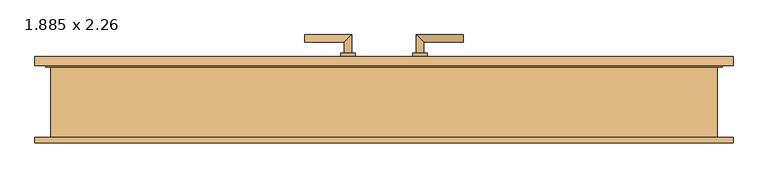
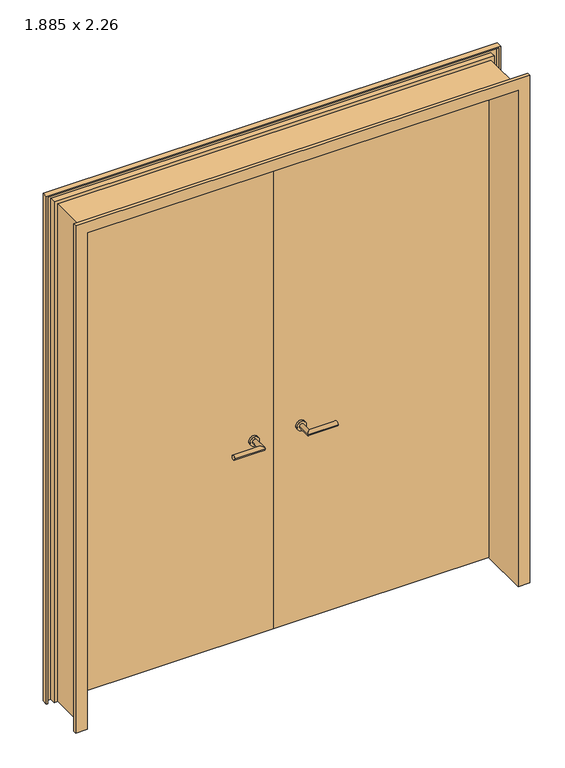
"""IFC4 building model written with IfcOpenShell, lengths in millimetres: door geometry, Drehflügel 2-flg - Stahlzarge : 1.885 x 2.26."""

from ifc_helpers import new_model, si_unit, point, frame, frame_2d, origin, place, context, project, spatial, polyline, circle_curve, ellipse_curve, trimmed, segment, composite_curve, outline, extrude, faceted_brep, source, transform, mapped, element, save
from ifc_brep_helpers import plane_surface, cylinder_surface, advanced_brep


def door_1_885_x_2_26_dae8c6c6(model_context):
    return source(origin(), model_context, "Body", "SolidModel", [
        advanced_brep(
        [(-90.0, 89.4346141, 1000.0), (-110.0, 89.4346141, 1000.0), (-110.0, 39.4346141, 1000.0), (-90.0, 19.4346141, 1000.0), (-220.0, 19.4346141, 1000.0), (-220.0, 39.4346141, 1000.0)],
        [
            (0, 1, circle_curve(frame((-100.0, 89.4346141, 1000.0), z_axis=(0.0, 1.0, 0.0), x_axis=(-1.0, 0.0, 0.0)), 10.0)),
            (1, 0, circle_curve(frame((-100.0, 89.4346141, 1000.0), z_axis=(0.0, 1.0, 0.0), x_axis=(-1.0, 0.0, 0.0)), 10.0)),
            (1, 2),
            (2, 3, ellipse_curve(frame((-100.0, 29.4346141, 1000.0), z_axis=(0.7071067811865385, 0.7071067811865565, 0.0), x_axis=(-0.7071067811865563, 0.7071067811865386, 0.0)), 14.1421356, 10.0)),
            (3, 0),
            (3, 2, ellipse_curve(frame((-100.0, 29.4346141, 1000.0), z_axis=(0.7071067811865385, 0.7071067811865565, 0.0), x_axis=(-0.7071067811865563, 0.7071067811865386, 0.0)), 14.1421356, 10.0)),
            (4, 5, circle_curve(frame((-220.0, 29.4346141, 1000.0), z_axis=(-1.0, 0.0, 0.0), x_axis=(0.0, 1.0, 0.0)), 10.0)),
            (5, 4, circle_curve(frame((-220.0, 29.4346141, 1000.0), z_axis=(-1.0, 0.0, 0.0), x_axis=(0.0, 1.0, 0.0)), 10.0)),
            (2, 5),
            (4, 3),
        ],
        [
            plane_surface(frame((-100.0, 89.4346141, -287.7526403), z_axis=(0.0, 1.0, 0.0), x_axis=(0.0, 0.0, 1.0))),
            cylinder_surface(frame((-100.0, 89.4346141, 1000.0), z_axis=(0.0, 1.0, 0.0), x_axis=(-1.0, 0.0, 0.0)), 10.0),
            plane_surface(frame((-220.0, 29.4346141, -287.7526403), z_axis=(-1.0, 0.0, 0.0), x_axis=(0.0, 0.0, 1.0))),
            cylinder_surface(frame((-100.0, 29.4346141, 1000.0), z_axis=(1.0, 0.0, 0.0), x_axis=(0.0, 1.0, 0.0)), 10.0),
        ],
        [
            (0, [[1, 2]]),
            (1, [[3, 4, 5, -2]]),
            (1, [[-5, 6, -3, -1]]),
            (2, [[7, 8]]),
            (3, [[9, -7, 10, -4]]),
            (3, [[-10, -8, -9, -6]]),
        ],
    ),
        advanced_brep(
        [(-110.0, 149.4346141, 1000.0), (-90.0, 149.4346141, 1000.0), (-90.0, 199.4346141, 1000.0), (-110.0, 179.4346141, 1000.0), (-220.0, 179.4346141, 1000.0), (-220.0, 199.4346141, 1000.0)],
        [
            (0, 1, circle_curve(frame((-100.0, 149.4346141, 1000.0), z_axis=(0.0, -1.0, 0.0), x_axis=(1.0, 0.0, 0.0)), 10.0)),
            (1, 0, circle_curve(frame((-100.0, 149.4346141, 1000.0), z_axis=(0.0, -1.0, 0.0), x_axis=(1.0, 0.0, 0.0)), 10.0)),
            (1, 2),
            (2, 3, ellipse_curve(frame((-100.0, 189.4346141, 1000.0), z_axis=(0.7071067811865475, -0.7071067811865475, 0.0), x_axis=(-0.7071067811865474, -0.7071067811865476, 0.0)), 14.1421356, 10.0)),
            (3, 0),
            (3, 2, ellipse_curve(frame((-100.0, 189.4346141, 1000.0), z_axis=(0.7071067811865475, -0.7071067811865475, 0.0), x_axis=(-0.7071067811865474, -0.7071067811865476, 0.0)), 14.1421356, 10.0)),
            (4, 5, circle_curve(frame((-220.0, 189.4346141, 1000.0), z_axis=(-1.0, 0.0, 0.0), x_axis=(0.0, 1.0, 0.0)), 10.0)),
            (5, 4, circle_curve(frame((-220.0, 189.4346141, 1000.0), z_axis=(-1.0, 0.0, 0.0), x_axis=(0.0, 1.0, 0.0)), 10.0)),
            (2, 5),
            (4, 3),
        ],
        [
            plane_surface(frame((-100.0, 149.4346141, -287.7526403), z_axis=(0.0, -1.0, 0.0), x_axis=(0.0, 0.0, 1.0))),
            cylinder_surface(frame((-100.0, 149.4346141, 1000.0), z_axis=(0.0, -1.0, 0.0), x_axis=(1.0, 0.0, 0.0)), 10.0),
            plane_surface(frame((-220.0, 189.4346141, -287.7526403), z_axis=(-1.0, 0.0, 0.0), x_axis=(0.0, 0.0, 1.0))),
            cylinder_surface(frame((-100.0, 189.4346141, 1000.0), z_axis=(1.0, 0.0, 0.0), x_axis=(0.0, 1.0, 0.0)), 10.0),
        ],
        [
            (0, [[1, 2]]),
            (1, [[3, 4, 5, -2]]),
            (1, [[-5, 6, -3, -1]]),
            (2, [[7, 8]]),
            (3, [[9, -7, 10, -4]]),
            (3, [[-10, -8, -9, -6]]),
        ],
    ),
        extrude(outline(composite_curve([segment(trimmed(circle_curve(frame_2d((1000.0, -100.0)), 20.0), [point((1000.0, -80.0))], [point((1000.0, -120.0))], False, "CARTESIAN"), True, "CONTINUOUS"), segment(trimmed(circle_curve(frame_2d((1000.0, -100.0)), 20.0), [point((1000.0, -120.0))], [point((1000.0, -80.0))], False, "CARTESIAN"), True, "CONTINUOUS")], self_intersect=False)), frame((0.0, 79.4346141, 0.0), z_axis=(0.0, 1.0, 0.0), x_axis=(0.0, 0.0, 1.0)), (0.0, 0.0, 1.0), 10.0),
        extrude(outline(composite_curve([segment(trimmed(circle_curve(frame_2d((1000.0, -100.0)), 20.0), [point((1000.0, -80.0))], [point((1000.0, -120.0))], False, "CARTESIAN"), True, "CONTINUOUS"), segment(trimmed(circle_curve(frame_2d((1000.0, -100.0)), 20.0), [point((1000.0, -120.0))], [point((1000.0, -80.0))], False, "CARTESIAN"), True, "CONTINUOUS")], self_intersect=False)), frame((0.0, 139.4346141, 0.0), z_axis=(0.0, 1.0, 0.0), x_axis=(0.0, 0.0, 1.0)), (0.0, 0.0, 1.0), 10.0),
        advanced_brep(
        [(90.0, 89.4346141, 1000.0), (110.0, 89.4346141, 1000.0), (90.0, 19.4346141, 1000.0), (110.0, 39.4346141, 1000.0), (220.0, 19.4346141, 1000.0), (220.0, 39.4346141, 1000.0)],
        [
            (0, 1, circle_curve(frame((100.0, 89.4346141, 1000.0), z_axis=(0.0, 1.0, 0.0), x_axis=(1.0, 0.0, 0.0)), 10.0)),
            (1, 0, circle_curve(frame((100.0, 89.4346141, 1000.0), z_axis=(0.0, 1.0, 0.0), x_axis=(1.0, 0.0, 0.0)), 10.0)),
            (0, 2),
            (2, 3, ellipse_curve(frame((100.0, 29.4346141, 1000.0), z_axis=(-0.7071067811865385, 0.7071067811865565, 0.0), x_axis=(0.7071067811865563, 0.7071067811865386, 0.0)), 14.1421356, 10.0)),
            (3, 1),
            (3, 2, ellipse_curve(frame((100.0, 29.4346141, 1000.0), z_axis=(-0.7071067811865385, 0.7071067811865565, 0.0), x_axis=(0.7071067811865563, 0.7071067811865386, 0.0)), 14.1421356, 10.0)),
            (4, 5, circle_curve(frame((220.0, 29.4346141, 1000.0), z_axis=(1.0, 0.0, 0.0), x_axis=(0.0, 1.0, 0.0)), 10.0)),
            (5, 4, circle_curve(frame((220.0, 29.4346141, 1000.0), z_axis=(1.0, 0.0, 0.0), x_axis=(0.0, 1.0, 0.0)), 10.0)),
            (2, 4),
            (5, 3),
        ],
        [
            plane_surface(frame((100.0, 89.4346141, -287.7526403), z_axis=(0.0, 1.0, 0.0), x_axis=(0.0, 0.0, 1.0))),
            cylinder_surface(frame((100.0, 89.4346141, 1000.0), z_axis=(0.0, 1.0, 0.0), x_axis=(1.0, 0.0, 0.0)), 10.0),
            plane_surface(frame((220.0, 29.4346141, -287.7526403), z_axis=(1.0, 0.0, 0.0), x_axis=(0.0, 0.0, 1.0))),
            cylinder_surface(frame((100.0, 29.4346141, 1000.0), z_axis=(-1.0, 0.0, 0.0), x_axis=(0.0, 1.0, 0.0)), 10.0),
        ],
        [
            (0, [[1, 2]]),
            (1, [[-1, 3, 4, 5]]),
            (1, [[-2, -5, 6, -3]]),
            (2, [[7, 8]]),
            (3, [[-4, 9, -8, 10]]),
            (3, [[-6, -10, -7, -9]]),
        ],
    ),
        advanced_brep(
        [(110.0, 149.4346141, 1000.0), (90.0, 149.4346141, 1000.0), (110.0, 179.4346141, 1000.0), (90.0, 199.4346141, 1000.0), (220.0, 179.4346141, 1000.0), (220.0, 199.4346141, 1000.0)],
        [
            (0, 1, circle_curve(frame((100.0, 149.4346141, 1000.0), z_axis=(0.0, -1.0, 0.0), x_axis=(-1.0, 0.0, 0.0)), 10.0)),
            (1, 0, circle_curve(frame((100.0, 149.4346141, 1000.0), z_axis=(0.0, -1.0, 0.0), x_axis=(-1.0, 0.0, 0.0)), 10.0)),
            (0, 2),
            (2, 3, ellipse_curve(frame((100.0, 189.4346141, 1000.0), z_axis=(-0.7071067811865475, -0.7071067811865475, 0.0), x_axis=(0.7071067811865474, -0.7071067811865476, 0.0)), 14.1421356, 10.0)),
            (3, 1),
            (3, 2, ellipse_curve(frame((100.0, 189.4346141, 1000.0), z_axis=(-0.7071067811865475, -0.7071067811865475, 0.0), x_axis=(0.7071067811865474, -0.7071067811865476, 0.0)), 14.1421356, 10.0)),
            (4, 5, circle_curve(frame((220.0, 189.4346141, 1000.0), z_axis=(1.0, 0.0, 0.0), x_axis=(0.0, 1.0, 0.0)), 10.0)),
            (5, 4, circle_curve(frame((220.0, 189.4346141, 1000.0), z_axis=(1.0, 0.0, 0.0), x_axis=(0.0, 1.0, 0.0)), 10.0)),
            (2, 4),
            (5, 3),
        ],
        [
            plane_surface(frame((100.0, 149.4346141, -287.7526403), z_axis=(0.0, -1.0, 0.0), x_axis=(0.0, 0.0, 1.0))),
            cylinder_surface(frame((100.0, 149.4346141, 1000.0), z_axis=(0.0, -1.0, 0.0), x_axis=(-1.0, 0.0, 0.0)), 10.0),
            plane_surface(frame((220.0, 189.4346141, -287.7526403), z_axis=(1.0, 0.0, 0.0), x_axis=(0.0, 0.0, 1.0))),
            cylinder_surface(frame((100.0, 189.4346141, 1000.0), z_axis=(-1.0, 0.0, 0.0), x_axis=(0.0, 1.0, 0.0)), 10.0),
        ],
        [
            (0, [[1, 2]]),
            (1, [[-1, 3, 4, 5]]),
            (1, [[-2, -5, 6, -3]]),
            (2, [[7, 8]]),
            (3, [[-4, 9, -8, 10]]),
            (3, [[-6, -10, -7, -9]]),
        ],
    ),
        extrude(outline(composite_curve([segment(trimmed(circle_curve(frame_2d((1000.0, 100.0)), 20.0), [point((1000.0, 80.0))], [point((1000.0, 120.0))], False, "CARTESIAN"), True, "CONTINUOUS"), segment(trimmed(circle_curve(frame_2d((1000.0, 100.0)), 20.0), [point((1000.0, 120.0))], [point((1000.0, 80.0))], False, "CARTESIAN"), True, "CONTINUOUS")], self_intersect=False)), frame((0.0, 79.4346141, 0.0), z_axis=(0.0, 1.0, 0.0), x_axis=(0.0, 0.0, 1.0)), (0.0, 0.0, 1.0), 10.0),
        extrude(outline(composite_curve([segment(trimmed(circle_curve(frame_2d((1000.0, 100.0)), 20.0), [point((1000.0, 80.0))], [point((1000.0, 120.0))], False, "CARTESIAN"), True, "CONTINUOUS"), segment(trimmed(circle_curve(frame_2d((1000.0, 100.0)), 20.0), [point((1000.0, 120.0))], [point((1000.0, 80.0))], False, "CARTESIAN"), True, "CONTINUOUS")], self_intersect=False)), frame((0.0, 139.4346141, 0.0), z_axis=(0.0, 1.0, 0.0), x_axis=(0.0, 0.0, 1.0)), (0.0, 0.0, 1.0), 10.0),
        extrude(outline(polyline([(0.0, 114.4346141), (-932.5, 114.4346141), (-932.5, 139.4346141), (0.0, 139.4346141), (0.0, 114.4346141)])), frame((0.0, 0.0, 100.0), z_axis=(0.0, 0.0, 1.0), x_axis=(1.0, 0.0, 0.0)), (0.0, 0.0, 1.0), 2250.0),
        extrude(outline(polyline([(932.5, 114.4346141), (0.0, 114.4346141), (0.0, 139.4346141), (932.5, 139.4346141), (932.5, 114.4346141)])), frame((0.0, 0.0, 100.0), z_axis=(0.0, 0.0, 1.0), x_axis=(1.0, 0.0, 0.0)), (0.0, 0.0, 1.0), 2250.0),
        faceted_brep([(967.0, -100.5653859, 100.0), (917.5, -100.5653859, 100.0), (917.5, 114.4346141, 100.0), (932.5, 114.4346141, 100.0), (932.5, 139.4346141, 100.0), (967.0, 139.4346141, 100.0), (967.0, 114.4346141, 100.0), (962.0, 114.4346141, 100.0), (962.0, 134.4346141, 100.0), (937.5, 134.4346141, 100.0), (937.5, 109.4346141, 100.0), (922.5, 109.4346141, 100.0), (922.5, -95.5653859, 100.0), (962.0, -95.5653859, 100.0), (962.0, -85.5653859, 100.0), (967.0, -85.5653859, 100.0), (967.0, -100.5653859, 2384.5), (-967.0, -100.5653859, 2384.5), (-967.0, -100.5653859, 100.0), (-917.5, -100.5653859, 100.0), (-917.5, -100.5653859, 2335.0), (917.5, -100.5653859, 2335.0), (917.5, 114.4346141, 2335.0), (-917.5, 114.4346141, 2335.0), (-917.5, 114.4346141, 100.0), (-932.5, 114.4346141, 100.0), (-932.5, 114.4346141, 2350.0), (932.5, 114.4346141, 2350.0), (932.5, 139.4346141, 2350.0), (-932.5, 139.4346141, 2350.0), (-932.5, 139.4346141, 100.0), (-967.0, 139.4346141, 100.0), (-967.0, 139.4346141, 2384.5), (967.0, 139.4346141, 2384.5), (967.0, 114.4346141, 2384.5), (-967.0, 114.4346141, 2384.5), (-967.0, 114.4346141, 100.0), (-962.0, 114.4346141, 100.0), (-962.0, 114.4346141, 2379.5), (962.0, 114.4346141, 2379.5), (962.0, 134.4346141, 2379.5), (-962.0, 134.4346141, 2379.5), (-962.0, 134.4346141, 100.0), (-937.5, 134.4346141, 100.0), (-937.5, 134.4346141, 2355.0), (937.5, 134.4346141, 2355.0), (937.5, 109.4346141, 2355.0), (-937.5, 109.4346141, 2355.0), (-937.5, 109.4346141, 100.0), (-922.5, 109.4346141, 100.0), (-922.5, 109.4346141, 2340.0), (922.5, 109.4346141, 2340.0), (922.5, -95.5653859, 2340.0), (-922.5, -95.5653859, 2340.0), (-922.5, -95.5653859, 100.0), (-962.0, -95.5653859, 100.0), (-962.0, -95.5653859, 2379.5), (962.0, -95.5653859, 2379.5), (962.0, -85.5653859, 2379.5), (-962.0, -85.5653859, 2379.5), (-962.0, -85.5653859, 100.0), (-967.0, -85.5653859, 100.0), (-967.0, -85.5653859, 2384.5), (967.0, -85.5653859, 2384.5)], [[[0, 1, 2, 3, 4, 5, 6, 7, 8, 9, 10, 11, 12, 13, 14, 15]], [[1, 0, 16, 17, 18, 19, 20, 21]], [[2, 1, 21, 22]], [[3, 2, 22, 23, 24, 25, 26, 27]], [[4, 3, 27, 28]], [[5, 4, 28, 29, 30, 31, 32, 33]], [[6, 5, 33, 34]], [[7, 6, 34, 35, 36, 37, 38, 39]], [[8, 7, 39, 40]], [[9, 8, 40, 41, 42, 43, 44, 45]], [[10, 9, 45, 46]], [[11, 10, 46, 47, 48, 49, 50, 51]], [[12, 11, 51, 52]], [[13, 12, 52, 53, 54, 55, 56, 57]], [[14, 13, 57, 58]], [[15, 14, 58, 59, 60, 61, 62, 63]], [[0, 15, 63, 16]], [[17, 62, 61, 18]], [[18, 61, 60, 55, 54, 49, 48, 43, 42, 37, 36, 31, 30, 25, 24, 19]], [[23, 20, 19, 24]], [[29, 26, 25, 30]], [[35, 32, 31, 36]], [[41, 38, 37, 42]], [[47, 44, 43, 48]], [[53, 50, 49, 54]], [[59, 56, 55, 60]], [[22, 21, 20, 23]], [[28, 27, 26, 29]], [[34, 33, 32, 35]], [[40, 39, 38, 41]], [[46, 45, 44, 47]], [[52, 51, 50, 53]], [[58, 57, 56, 59]], [[16, 63, 62, 17]]]),
    ])


if __name__ == "__main__":
    model = new_model("IFC4")
    model_context = context("Model", 3, world=origin())
    ifc_project = project(units=[si_unit("LENGTHUNIT", "METRE", prefix="MILLI")], contexts=[model_context])
    site = spatial("IfcSite", under=ifc_project)
    building = spatial("IfcBuilding", under=site)
    placement = place(None, origin())
    door_1_885_x_2_26_shape = door_1_885_x_2_26_dae8c6c6(model_context)
    element("IfcDoor", 1, ObjectType="Drehflügel 2-flg - Stahlzarge : 1.885 x 2.26", at=placement, inside=building, context=model_context, shape_type="MappedRepresentation", body=[
        mapped(door_1_885_x_2_26_shape, transform((0.0, 0.0, 0.0), x_axis=(1.0, 0.0, 0.0), y_axis=(0.0, 1.0, 0.0), z_axis=(0.0, 0.0, 1.0))),
    ])
    save(model, "model.ifc")

# Revit data of these elements
# Type "Drehflügel 2-flg - Stahlzarge : 1.885 x 2.26"
#   Construction Type Id = "MDOOR"
#   Type Mark = "19"
#   Operation = "DoubleDoorSingleSwing"
#   Keynote = "16.03"
#   Analytic Construction = "Metall"
#   Thermal Resistance (R) = 0.270117 (m²·K)/W
#   Heat Transfer Coefficient (U) = 3.7021 W/(m²·K)
#   Rough Width = 1.885 m
#   Rough Height [instance default] = 2.360 m
#   Höhe Türgriff = 0.900 m
#   Height = 2.260 m
#   Fußbodenaufbau [instance default] = 0.100 m
#   Width = 1.885 m
#   Sichtbarkeit Sturzlinien [instance default] = yes
#   Türgriff auswählen [instance default] = element 219327
#   Türgriff [instance default] = none
#   Türflügel [instance default] = none
#   Rahmen/Pfosten [instance default] = Metall - Lackiert - Grau
#   Visual Light Transmittance = 0
#   Solar Heat Gain Coefficient = 0
#   Function = (empty or 0)
#   Wall Closure = (empty or 0)
# Element 1 (IfcDoor, "Drehflügel 2-flg - Stahlzarge : 1.885 x 2.26")
#   Materials on its faces: "Metall - Chrom", "Metall - Lackiert - Grau", "Holz - Birke"
# Materials
#   "Metall - Lackiert - Grau": class "Farbe 1", colour RGB 98 98 98, transparency 0, Cost = 0
#   "Metall - Chrom": class "Metall", colour RGB 247 247 247, transparency 0, Cost = 0
#   "Holz - Birke": class "Holz", colour RGB 213 164 103, transparency 0, Cost = 0
